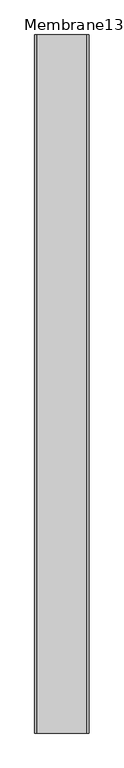
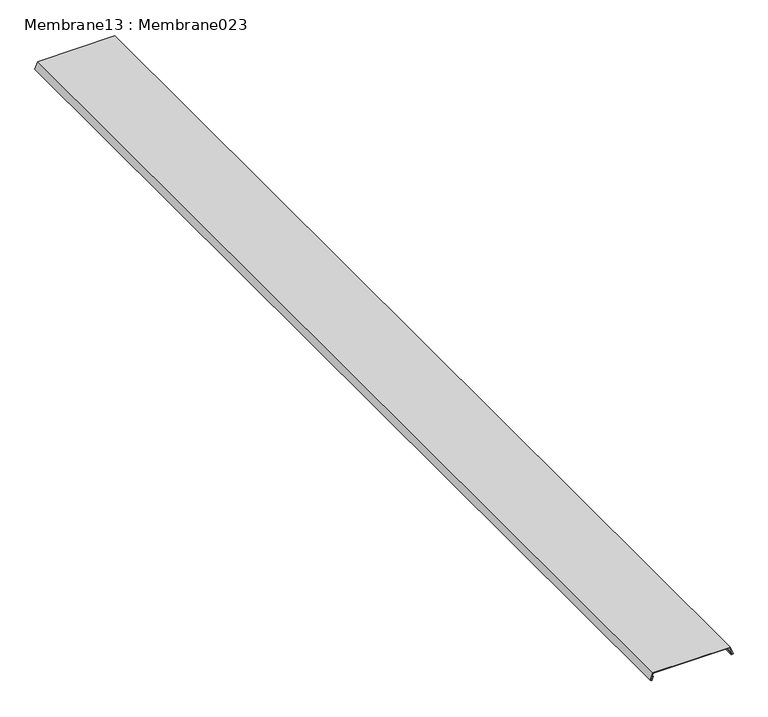
"""IFC4 building model written with IfcOpenShell, lengths in millimetres: proxy geometry, Membrane13 : Membrane023."""

from ifc_helpers import new_model, si_unit, frame, origin, place, context, project, spatial, polyline, outline, extrude, source, transform, mapped, element, save


def membrane13_membrane023_074b6dce(model_context):
    return source(origin(), model_context, "Body", "SweptSolid", [
        extrude(outline(polyline([(40125.2594856, -9579.4752528), (40125.2594856, -9724.6705583), (40111.4755464, -9729.6875019), (40110.2712379, -9726.3786915), (40117.4400699, -9723.76945), (40117.7820901, -9724.7091426), (40111.5529506, -9726.9763639), (40112.0732189, -9728.4057891), (40124.2594856, -9723.9703507), (40124.2594856, -9580.1754603), (40110.4916524, -9575.1643789), (40109.9713842, -9576.593804), (40116.2005236, -9578.8610254), (40115.8585035, -9579.800718), (40108.6896714, -9577.1914765), (40109.8939799, -9573.8826661), (40125.2594856, -9579.4752528)])), frame((0.0, 7182.1531721, 0.0), z_axis=(0.0, 1.0, 0.0), x_axis=(0.0, 0.0, 1.0)), (0.0, 0.0, 1.0), 2000.0),
    ])


if __name__ == "__main__":
    model = new_model("IFC4")
    model_context = context("Model", 3, world=origin())
    ifc_project = project(units=[si_unit("LENGTHUNIT", "METRE", prefix="MILLI")], contexts=[model_context])
    site = spatial("IfcSite", under=ifc_project)
    building = spatial("IfcBuilding", under=site)
    placement = place(None, origin())
    membrane13_membrane023_shape = membrane13_membrane023_074b6dce(model_context)
    element("IfcBuildingElementProxy", 1, Name="Membrane13 : Membrane023", ObjectType="Membrane13 : Membrane023", at=placement, inside=building, context=model_context, shape_type="MappedRepresentation", body=[
        mapped(membrane13_membrane023_shape, transform((0.0, 0.0, 0.0), x_axis=(1.0, 0.0, 0.0), y_axis=(0.0, 1.0, 0.0), z_axis=(0.0, 0.0, 1.0))),
    ])
    save(model, "model.ifc")

# Revit data of these elements
# Type "Membrane13 : Membrane023"
#   NameOverride = "Membrane023"
# Element 1 (IfcBuildingElementProxy, "Membrane13 : Membrane023")
#   Materials on its faces: "16 GA. COPPER FLASHING"
# Materials
#   "16 GA. COPPER FLASHING": class "Unassigned", colour RGB 251 232 155, transparency 0, Cost = 0
